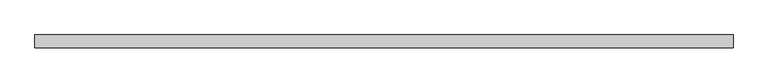
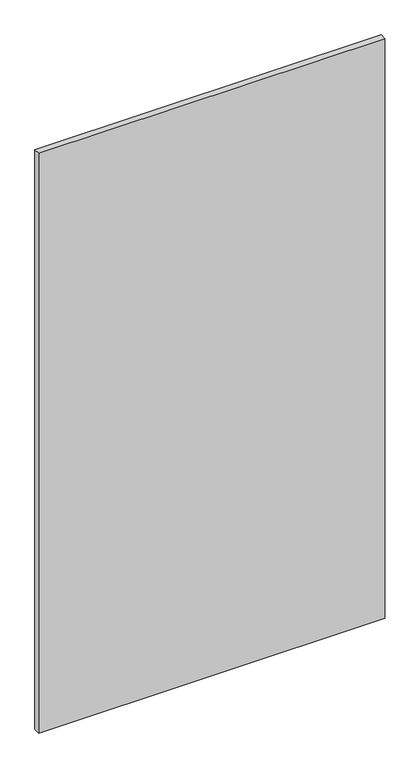
"""IFC4 building model written with IfcOpenShell, lengths in millimetres: plate geometry, システム パネル : ガラス."""

from ifc_helpers import new_model, si_unit, origin, origin_with_axes, place, context, project, spatial, polyline, outline, extrude, source, transform, mapped, element, save


def plate_c1c025ea(model_context):
    return source(origin(), model_context, "Body", "SweptSolid", [
        extrude(outline(polyline([(678.1250001, 24.5), (-678.1250001, 24.5), (-678.1250001, 49.5), (678.1250001, 49.5), (678.1250001, 24.5)])), origin_with_axes(), (0.0, 0.0, 1.0), 2400.0),
    ])


if __name__ == "__main__":
    model = new_model("IFC4")
    model_context = context("Model", 3, world=origin())
    ifc_project = project(units=[si_unit("LENGTHUNIT", "METRE", prefix="MILLI")], contexts=[model_context])
    site = spatial("IfcSite", under=ifc_project)
    building = spatial("IfcBuilding", under=site)
    placement = place(None, origin())
    plate_shape = plate_c1c025ea(model_context)
    element("IfcPlate", 1, ObjectType="システム パネル : ガラス", at=placement, inside=building, context=model_context, shape_type="MappedRepresentation", body=[
        mapped(plate_shape, transform((0.0, 0.0, 0.0), x_axis=(1.0, 0.0, 0.0), y_axis=(0.0, 1.0, 0.0), z_axis=(0.0, 0.0, 1.0))),
    ])
    save(model, "model.ifc")

# Revit data of these elements
# Type "システム パネル : ガラス"
#   Construction Type Id = "GSP4R"
#   Analytic Construction = "1/8 インチ ピルキントン一重ガラス"
#   Visual Light Transmittance = 0.9
#   Solar Heat Gain Coefficient = 0.86
#   Heat Transfer Coefficient (U) = 6.7069 W/(m²·K)
# Element 1 (IfcPlate, "システム パネル : ガラス")
#   Materials on its faces: "ガラス - 透明"
# Materials
#   "ガラス - 透明": class "ガラス", colour RGB 0 128 192, transparency 0.9, Cost = 0
